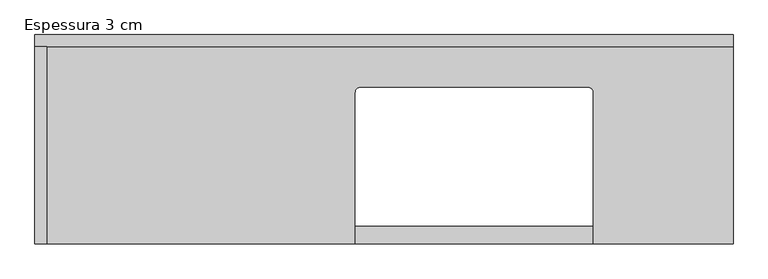
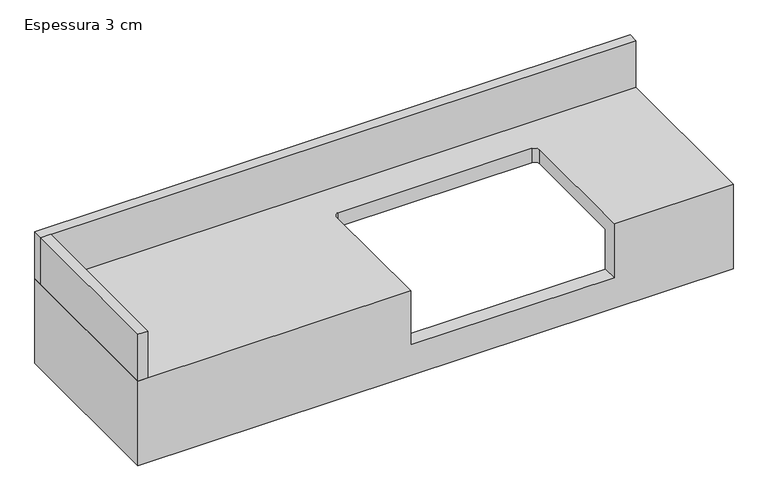
"""IFC4 building model written with IfcOpenShell, lengths in millimetres: furniture geometry, CC_BANCADA BANHEIRO COM CUBA_CANTO RETO : Espessura 3 cm."""

import ifcopenshell
import ifcopenshell.guid

model = None  # the IFC model being written
_history = None  # IfcOwnerHistory: only IFC2X3 demands one
_inside = {}  # id of a spatial element -> (the spatial element, [elements in it])
_under = {}  # id of a project, library or spatial element -> (it, [spatial elements below it])
_declared = {}  # id of a project -> (the project, [libraries it declares])
_typed = {}  # id of a type object -> (the type object, [elements of that type])
_made_of = {}  # id of a material, layer set ... -> (it, [elements and type objects made of it])


def new_model(schema):
    """Start an empty IFC model of exactly this schema.

    Asked for "IFC4X3", IfcOpenShell would pick the latest addendum, in which some entities
    have other attributes; the version numbers below select the first issue.
    IFC2X3 requires an IfcOwnerHistory on every rooted entity: one is made here for all.
    """
    global model, _history
    if schema == "IFC4X3":
        model = ifcopenshell.file(schema_version=(4, 3, 0, 0))
    else:
        model = ifcopenshell.file(schema=schema)
    _inside.clear()
    _under.clear()
    _declared.clear()
    _typed.clear()
    _made_of.clear()
    _history = None
    if model.schema == "IFC2X3":
        org = make("IfcOrganization", Name="unknown")
        user = make(
            "IfcPersonAndOrganization",
            ThePerson=make("IfcPerson", FamilyName="unknown"),
            TheOrganization=org,
        )
        app = make(
            "IfcApplication",
            ApplicationDeveloper=org,
            Version="unknown",
            ApplicationFullName="unknown",
            ApplicationIdentifier="unknown",
        )
        _history = make(
            "IfcOwnerHistory",
            OwningUser=user,
            OwningApplication=app,
            ChangeAction="ADDED",
            CreationDate=0,
        )
    return model


def make(cls, **values):
    """One entity of the class cls with the attributes given. An attribute that is None is left unset."""
    return model.create_entity(
        cls, **{name: value for name, value in values.items() if value is not None}
    )


def rooted(cls, **values):
    """An entity with a GlobalId (a new one), such as an element, a storey or a relation."""
    return make(cls, GlobalId=ifcopenshell.guid.new(), OwnerHistory=_history, **values)


def si_unit(unit_type, name, prefix=None):
    """IfcSIUnit, for example si_unit("LENGTHUNIT", "METRE", prefix="MILLI")."""
    return make("IfcSIUnit", UnitType=unit_type, Prefix=prefix, Name=name)


def assignment(units):
    """IfcUnitAssignment: the units of a project."""
    return None if units is None else make("IfcUnitAssignment", Units=units)


def point(xyz):
    """IfcCartesianPoint."""
    return None if xyz is None else make("IfcCartesianPoint", Coordinates=xyz)


def direction(xyz):
    """IfcDirection."""
    return None if xyz is None else make("IfcDirection", DirectionRatios=xyz)


def frame(location, z_axis=None, x_axis=None):
    """IfcAxis2Placement3D, a coordinate frame: its origin and axes. An axis left out is left unset."""
    return make(
        "IfcAxis2Placement3D",
        Location=point(location),
        Axis=direction(z_axis),
        RefDirection=direction(x_axis),
    )


def origin():
    """The frame at (0, 0, 0) with its axes left unset."""
    return frame((0.0, 0.0, 0.0))


def place(relative_to, where):
    """IfcLocalPlacement: puts the frame where relative to a parent placement (None: the world)."""
    return make(
        "IfcLocalPlacement", PlacementRelTo=relative_to, RelativePlacement=where
    )


def context(
    kind, dimensions, precision=None, world=None, true_north=None, identifier=None
):
    """IfcGeometricRepresentationContext, for example the 3D "Model" context."""
    return make(
        "IfcGeometricRepresentationContext",
        ContextIdentifier=identifier,
        ContextType=kind,
        CoordinateSpaceDimension=dimensions,
        Precision=precision,
        WorldCoordinateSystem=world,
        TrueNorth=true_north,
    )


def project(units=None, contexts=None):
    """IfcProject with its units and contexts."""
    return rooted(
        "IfcProject",
        Name="project",
        RepresentationContexts=contexts,
        UnitsInContext=assignment(units),
    )


def spatial(cls, under=None, at=None, **own):
    """A site, building, storey or space (cls), placed at a placement, below another one or the project."""
    s = rooted(cls, ObjectPlacement=at, **own)
    if under is not None:
        _under.setdefault(under.id(), (under, []))[1].append(s)
    return s


def polyline(points):
    """IfcPolyline through the points."""
    return make("IfcPolyline", Points=[point(p) for p in points])


def circle_curve(where, radius):
    """IfcCircle in the frame where."""
    return make("IfcCircle", Position=where, Radius=radius)


def outline(outer, holes=None, kind="AREA"):
    """IfcArbitraryClosedProfileDef: a profile drawn as a closed curve; with holes, ...WithVoids."""
    if holes is None:
        return make("IfcArbitraryClosedProfileDef", ProfileType=kind, OuterCurve=outer)
    return make(
        "IfcArbitraryProfileDefWithVoids",
        ProfileType=kind,
        OuterCurve=outer,
        InnerCurves=holes,
    )


def extrude(swept, where, along, depth):
    """IfcExtrudedAreaSolid: the profile swept, set in the frame where, extruded along a direction by depth."""
    return make(
        "IfcExtrudedAreaSolid",
        SweptArea=swept,
        Position=where,
        ExtrudedDirection=direction(along),
        Depth=depth,
    )


def shape(context_of_items, identifier, shape_type, items):
    """IfcShapeRepresentation: the items that make up one representation, for example the "Body"."""
    return make(
        "IfcShapeRepresentation",
        ContextOfItems=context_of_items,
        RepresentationIdentifier=identifier,
        RepresentationType=shape_type,
        Items=items,
    )


def source(mapping_origin, context_of_items, identifier, shape_type, items):
    """IfcRepresentationMap: a shape defined once, which mapped items show again and again."""
    return make(
        "IfcRepresentationMap",
        MappingOrigin=mapping_origin,
        MappedRepresentation=shape(context_of_items, identifier, shape_type, items),
    )


def transform(
    local_origin,
    x_axis=None,
    y_axis=None,
    z_axis=None,
    scale=None,
    scale2=None,
    scale3=None,
    uniform=True,
):
    """IfcCartesianTransformationOperator3D, or its non-uniform kind. x_axis, y_axis, z_axis: its Axis1, 2, 3."""
    if uniform:
        return make(
            "IfcCartesianTransformationOperator3D",
            Axis1=direction(x_axis),
            Axis2=direction(y_axis),
            LocalOrigin=point(local_origin),
            Scale=scale,
            Axis3=direction(z_axis),
        )
    return make(
        "IfcCartesianTransformationOperator3DnonUniform",
        Axis1=direction(x_axis),
        Axis2=direction(y_axis),
        LocalOrigin=point(local_origin),
        Scale=scale,
        Axis3=direction(z_axis),
        Scale2=scale2,
        Scale3=scale3,
    )


def mapped(mapping_source, mapping_target):
    """IfcMappedItem: shows the shape of a source again, moved by a transform."""
    return make(
        "IfcMappedItem", MappingSource=mapping_source, MappingTarget=mapping_target
    )


def made_of(thing, what):
    """Note that an element or type object is made of a material, layer set ...; save() writes the relation."""
    if what is not None:
        _made_of.setdefault(what.id(), (what, []))[1].append(thing)
    return thing


def element(
    cls,
    number,
    at=None,
    inside=None,
    cuts=None,
    type_object=None,
    material=None,
    context=None,
    identifier="Body",
    shape_type=None,
    held_by="IfcProductDefinitionShape",
    body=None,
    shapes=None,
    **own,
):
    """One element of the class cls, such as IfcWall. Its Tag is "e" and its number.

    at: its placement. inside: the storey or other place that contains it. cuts: it is an
    opening in that element (IfcRelVoidsElement). A single representation is given by context,
    identifier, shape_type and body (its items); several are given by shapes. held_by: the class
    of the entity that holds the representations. save() writes the other relations.
    """
    e = rooted(cls, Tag="e%d" % number, ObjectPlacement=at, **own)
    if body is not None:
        shapes = [shape(context, identifier, shape_type, body)]
    if shapes is not None:
        e.Representation = make(held_by, Representations=shapes)
    if inside is not None:
        _inside.setdefault(inside.id(), (inside, []))[1].append(e)
    if cuts is not None:
        rooted(
            "IfcRelVoidsElement", RelatingBuildingElement=cuts, RelatedOpeningElement=e
        )
    if type_object is not None:
        _typed.setdefault(type_object.id(), (type_object, []))[1].append(e)
    return made_of(e, material)


def aggregate(whole, parts):
    """IfcRelAggregates: a whole, such as a stair, and the parts it consists of."""
    return rooted("IfcRelAggregates", RelatingObject=whole, RelatedObjects=parts)


def save(model, path):
    """Write the relations noted so far, then the file.

    IfcRelAggregates (storeys below a building ...), IfcRelContainedInSpatialStructure (elements
    in a storey), IfcRelDefinesByType, IfcRelAssociatesMaterial and IfcRelDeclares: one each for
    every whole, place, type object, material and project.
    """
    for whole, parts in _under.values():
        aggregate(whole, parts)
    for where, things in _inside.values():
        rooted(
            "IfcRelContainedInSpatialStructure",
            RelatedElements=things,
            RelatingStructure=where,
        )
    for kind, things in _typed.values():
        rooted("IfcRelDefinesByType", RelatedObjects=things, RelatingType=kind)
    for what, things in _made_of.values():
        rooted("IfcRelAssociatesMaterial", RelatedObjects=things, RelatingMaterial=what)
    for by, libraries in _declared.values():
        rooted("IfcRelDeclares", RelatingContext=by, RelatedDefinitions=libraries)
    model.write(path)


def plane_surface(at):
    """IfcPlane: the flat surface through the origin of the frame at, square to its z axis."""
    return make("IfcPlane", Position=at)


def revolved_surface(curve, axis_point, axis_direction):
    """IfcSurfaceOfRevolution: the curve turned about the line through axis_point along axis_direction."""
    return make(
        "IfcSurfaceOfRevolution",
        SweptCurve=make("IfcArbitraryOpenProfileDef", ProfileType="CURVE", Curve=curve),
        AxisPosition=make("IfcAxis1Placement", Location=point(axis_point), Axis=direction(axis_direction)),
    )


def advanced_brep(points, edges, surfaces, faces):
    """IfcAdvancedBrep: a solid bounded by faces that lie on surfaces and meet in shared edges.

    An edge is (start, end): straight between two places in points (the first is 0);
    or (start, end, curve); or (start, end, curve, False) where it runs against its curve.
    A face is (place in surfaces, loops), or (place, loops, False) where it looks against
    its surface's normal. A loop lists edges by number (the first is 1), with a minus sign
    where the edge is run from its end to its start. The first loop is the outer one.
    """
    corners = [point(p) for p in points]
    vertices = [make("IfcVertexPoint", VertexGeometry=c) for c in corners]
    made = []
    for start, end, *more in edges:
        made.append(
            make(
                "IfcEdgeCurve",
                EdgeStart=vertices[start],
                EdgeEnd=vertices[end],
                EdgeGeometry=more[0] if more else make("IfcPolyline", Points=[corners[start], corners[end]]),
                SameSense=more[1] if len(more) > 1 else True,
            )
        )
    hull = []
    for where, loops, *sense in faces:
        bounds = []
        for j, loop in enumerate(loops):
            ring = [make("IfcOrientedEdge", EdgeElement=made[abs(k) - 1], Orientation=k > 0) for k in loop]
            bounds.append(
                make(
                    "IfcFaceOuterBound" if j == 0 else "IfcFaceBound",
                    Bound=make("IfcEdgeLoop", EdgeList=ring),
                    Orientation=True,
                )
            )
        hull.append(make("IfcAdvancedFace", Bounds=bounds, FaceSurface=surfaces[where], SameSense=sense[0] if sense else True))
    return make("IfcAdvancedBrep", Outer=make("IfcClosedShell", CfsFaces=hull))


def espessura_3_cm_3b31cb49(model_context):
    return source(origin(), model_context, "Body", "SolidModel", [
        advanced_brep(
        [(750.0, 300.0, 860.0), (-450.0, 300.0, 860.0), (-450.0, -60.0, 860.0), (100.0, -60.0, 860.0), (100.0, 200.0, 860.0), (110.0, 210.0, 860.0), (500.0, 210.0, 860.0), (510.0, 200.0, 860.0), (510.0, -60.0, 860.0), (750.0, -60.0, 860.0), (750.0, 300.0, 680.0), (720.0, 300.0, 680.0), (720.0, 300.0, 830.0), (-420.0, 300.0, 830.0), (-420.0, 300.0, 680.0), (-450.0, 300.0, 680.0), (-450.0, -60.0, 680.0), (750.0, -60.0, 680.0), (510.0, -60.0, 745.0), (100.0, -60.0, 745.0), (720.0, -30.0, 830.0), (510.0, -30.0, 830.0), (510.0, 200.0, 830.0), (500.0, 210.0, 830.0), (110.0, 210.0, 830.0), (100.0, 200.0, 830.0), (100.0, -30.0, 830.0), (-420.0, -30.0, 830.0), (-420.0, -30.0, 680.0), (100.0, -30.0, 745.0), (510.0, -30.0, 745.0), (720.0, -30.0, 680.0)],
        [
            (0, 1),
            (1, 2),
            (2, 3),
            (3, 4),
            (4, 5, circle_curve(frame((110.0, 200.0, 860.0), z_axis=(0.0, 0.0, -1.0), x_axis=(0.0, 1.0, 0.0)), 10.0)),
            (5, 6),
            (6, 7, circle_curve(frame((500.0, 200.0, 860.0), z_axis=(0.0, 0.0, -1.0), x_axis=(0.0, 1.0, 0.0)), 10.0)),
            (7, 8),
            (8, 9),
            (9, 0),
            (0, 10),
            (10, 11),
            (11, 12),
            (12, 13),
            (13, 14),
            (14, 15),
            (15, 1),
            (15, 16),
            (16, 2),
            (16, 17),
            (17, 9),
            (8, 18),
            (18, 19),
            (19, 3),
            (17, 10),
            (12, 20),
            (20, 21),
            (21, 22),
            (22, 23, circle_curve(frame((500.0, 200.0, 830.0), z_axis=(0.0, 0.0, 1.0), x_axis=(0.0, 1.0, 0.0)), 10.0)),
            (23, 24),
            (24, 25, circle_curve(frame((110.0, 200.0, 830.0), z_axis=(0.0, 0.0, 1.0), x_axis=(0.0, 1.0, 0.0)), 10.0)),
            (25, 26),
            (26, 27),
            (27, 13),
            (27, 28),
            (28, 14),
            (26, 29),
            (29, 30),
            (30, 21),
            (20, 31),
            (31, 28),
            (11, 31),
            (5, 24),
            (23, 6),
            (18, 30),
            (29, 19),
            (4, 25),
            (7, 22),
        ],
        [
            plane_surface(frame((-450.0, 300.0, 860.0), z_axis=(0.0, 0.0, 1.0), x_axis=(-1.0, 0.0, 0.0))),
            plane_surface(frame((750.0, 300.0, 860.0), z_axis=(0.0, 1.0, 0.0), x_axis=(0.0, 0.0, -1.0))),
            plane_surface(frame((-450.0, 300.0, 860.0), z_axis=(-1.0, 0.0, 0.0), x_axis=(0.0, 0.0, -1.0))),
            plane_surface(frame((-450.0, -60.0, 860.0), z_axis=(0.0, -1.0, 0.0), x_axis=(0.0, 0.0, -1.0))),
            plane_surface(frame((750.0, -60.0, 860.0), z_axis=(1.0, 0.0, 0.0), x_axis=(0.0, 0.0, -1.0))),
            plane_surface(frame((-420.0, 300.0, 830.0), z_axis=(0.0, 0.0, -1.0), x_axis=(-1.0, 0.0, 0.0))),
            plane_surface(frame((-420.0, 300.0, 830.0), z_axis=(1.0, 0.0, 0.0), x_axis=(0.0, 0.0, -1.0))),
            plane_surface(frame((-420.0, -30.0, 830.0), z_axis=(0.0, 1.0, 0.0), x_axis=(0.0, 0.0, -1.0))),
            plane_surface(frame((720.0, -30.0, 830.0), z_axis=(-1.0, 0.0, 0.0), x_axis=(0.0, 0.0, -1.0))),
            plane_surface(frame((750.0, -60.0, 680.0), z_axis=(0.0, 0.0, -1.0), x_axis=(0.0, 1.0, 0.0))),
            plane_surface(frame((110.0, 210.0, 745.0), z_axis=(0.0, -1.0, 0.0), x_axis=(0.0, 0.0, 1.0))),
            plane_surface(frame((500.0, 210.0, 745.0), z_axis=(0.0, 0.0, 1.0), x_axis=(1.0, 0.0, 0.0))),
            revolved_surface(polyline([(110.0, 210.0, 830.0), (110.0, 210.0, 860.0)]), (110.0, 200.0, 900.0), (0.0, 0.0, -1.0)),
            plane_surface(frame((100.0, -190.0, 745.0), z_axis=(1.0, 0.0, 0.0), x_axis=(0.0, 0.0, 1.0))),
            plane_surface(frame((510.0, 200.0, 745.0), z_axis=(-1.0, 0.0, 0.0), x_axis=(0.0, 0.0, 1.0))),
            revolved_surface(polyline([(500.0, 210.0, 830.0), (500.0, 210.0, 860.0)]), (500.0, 200.0, 900.0), (0.0, 0.0, -1.0)),
        ],
        [
            (0, [[1, 2, 3, 4, 5, 6, 7, 8, 9, 10]]),
            (1, [[-1, 11, 12, 13, 14, 15, 16, 17]]),
            (2, [[-2, -17, 18, 19]]),
            (3, [[-3, -19, 20, 21, -9, 22, 23, 24]]),
            (4, [[-10, -21, 25, -11]]),
            (5, [[26, 27, 28, 29, 30, 31, 32, 33, 34, -14]]),
            (6, [[-34, 35, 36, -15]]),
            (7, [[-33, 37, 38, 39, -27, 40, 41, -35]]),
            (8, [[-26, -13, 42, -40]]),
            (9, [[-12, -25, -20, -18, -16, -36, -41, -42]]),
            (10, [[-6, 43, -30, 44]]),
            (11, [[-23, 45, -38, 46]]),
            (12, [[-5, 47, -31, -43]]),
            (13, [[-4, -24, -46, -37, -32, -47]]),
            (14, [[-8, 48, -28, -39, -45, -22]]),
            (15, [[-7, -44, -29, -48]]),
        ],
    ),
        extrude(outline(polyline([(-430.0, -60.0), (-450.0, -60.0), (-450.0, 280.0), (-430.0, 280.0), (-430.0, -60.0)])), frame((0.0, 0.0, 860.0), z_axis=(0.0, 0.0, 1.0), x_axis=(1.0, 0.0, 0.0)), (0.0, 0.0, 1.0), 100.0),
        extrude(outline(polyline([(750.0, 300.0), (750.0, 280.0), (-450.0, 280.0), (-450.0, 300.0), (750.0, 300.0)])), frame((0.0, 0.0, 860.0), z_axis=(0.0, 0.0, 1.0), x_axis=(1.0, 0.0, 0.0)), (0.0, 0.0, 1.0), 100.0),
    ])


if __name__ == "__main__":
    model = new_model("IFC4")
    model_context = context("Model", 3, world=origin())
    ifc_project = project(units=[si_unit("LENGTHUNIT", "METRE", prefix="MILLI")], contexts=[model_context])
    site = spatial("IfcSite", under=ifc_project)
    building = spatial("IfcBuilding", under=site)
    placement = place(None, origin())
    espessura_3_cm_shape = espessura_3_cm_3b31cb49(model_context)
    element("IfcFurniture", 1, ObjectType="CC_BANCADA BANHEIRO COM CUBA_CANTO RETO : Espessura 3 cm", at=placement, inside=building, context=model_context, shape_type="MappedRepresentation", body=[
        mapped(espessura_3_cm_shape, transform((0.0, 0.0, 0.0), x_axis=(1.0, 0.0, 0.0), y_axis=(0.0, 1.0, 0.0), z_axis=(0.0, 0.0, 1.0))),
    ])
    save(model, "model.ifc")

# Revit data of these elements
# Type "CC_BANCADA BANHEIRO COM CUBA_CANTO RETO : Espessura 3 cm"
#   Uso HS [instance default] = ""
#   h TESTEIRA AUX [instance default] = 0.15 m
#   Altura testeira [instance default] = 0.15 m
#   Altura rodapia [instance default] = 0.10 m
#   Espessura rodapia [instance default] = 0.02 m
#   Prof/2 [instance default] = 0.20 m
#   Offset cuba esquerda [instance default] = 0.40 m
#   Depth [instance default] = 1.20 m
#   Width [instance default] = 0.40 m
#   Espessura bancada = 0.03 m
#   Comprimento [instance default] = 1.20 m
#   Height [instance default] = 0.86 m
#   Testeira [instance default] = yes
#   Rodapia fundo [instance default] = no
#   Rodapia esquerda [instance default] = no
#   Rodapia direita [instance default] = no
#   Material porta-toalha [instance default] = .CROMADO
#   Material hidráulico [instance default] = .CROMADO
#   Material cuba [instance default] = .PORCELANA BRANCA
#   Material bancada [instance default] = .GRANITO_BRANCO_ITAUNAS
#   Assembly Code = ""
# Element 1 (IfcFurniture, "CC_BANCADA BANHEIRO COM CUBA_CANTO RETO : Espessura 3 cm")
#   Uso HS = "LAVABO"
#   Prof/2 = 0.18 m
#   Offset cuba esquerda = 0.55 m
#   Width = 0.36 m
#   Rodapia fundo = yes
#   Rodapia esquerda = yes
#   Materials on its faces: ".GRANITO_BRANCO_ITAUNAS"
# Materials
#   ".CROMADO": class "CC_METAIS", colour RGB 211 223 226, transparency 0, Cost = 0
#   ".PORCELANA BRANCA": class "CC_PORCELANA", colour RGB 230 230 230, transparency 0, Cost = 0
#   ".GRANITO_BRANCO_ITAUNAS": class ".CC_PEDRA REVEST.", colour RGB 202 195 174, transparency 0, Description = "Revestimento em granito", Cost = 0
